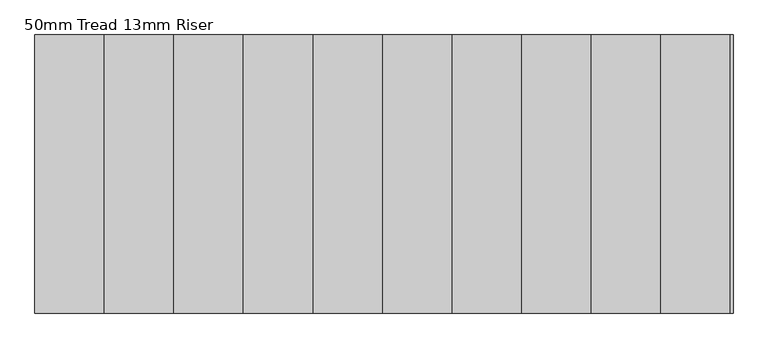
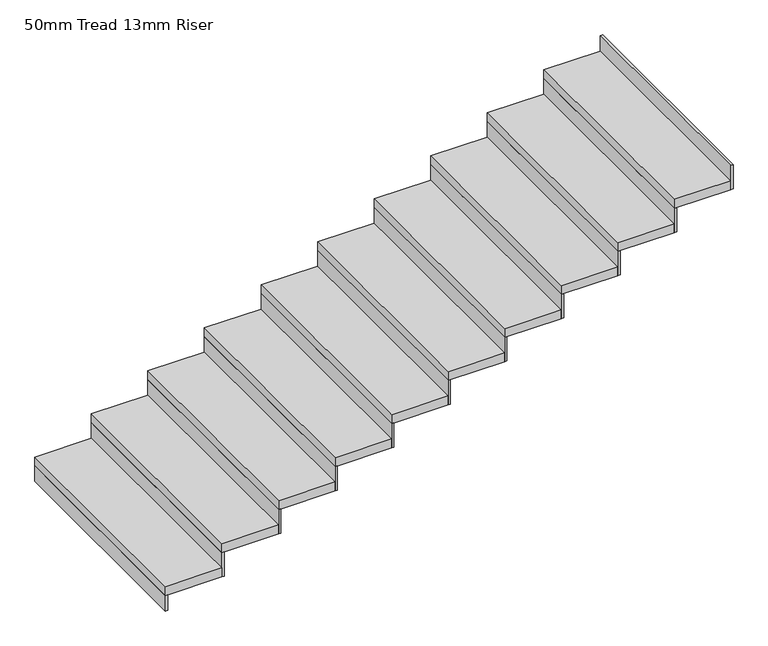
"""IFC4 building model written with IfcOpenShell, lengths in millimetres: stair flight geometry, 50mm Tread 13mm Riser."""

from ifc_helpers import new_model, si_unit, frame, origin, origin_with_axes, place, context, project, spatial, polyline, outline, extrude, source, transform, mapped, element, save


def stair_flight_50mm_tread_13mm_riser_f56aad4f(model_context):
    return source(origin(), model_context, "Body", "SweptSolid", [
        extrude(outline(polyline([(-12061.9417114, -7269.8807746), (-12074.4417114, -7269.8807746), (-12074.4417114, -6069.8807746), (-12061.9417114, -6069.8807746), (-12061.9417114, -7269.8807746)])), origin_with_axes(), (0.0, 0.0, 1.0), 86.3636364),
        extrude(outline(polyline([(-11774.4417114, -6069.8807746), (-11774.4417114, -7269.8807746), (-12074.4417114, -7269.8807746), (-12074.4417114, -6069.8807746), (-11774.4417114, -6069.8807746)])), frame((0.0, 0.0, 86.3636364), z_axis=(0.0, 0.0, 1.0), x_axis=(1.0, 0.0, 0.0)), (0.0, 0.0, 1.0), 50.0),
        extrude(outline(polyline([(-11761.9417114, -7269.8807746), (-11774.4417114, -7269.8807746), (-11774.4417114, -6069.8807746), (-11761.9417114, -6069.8807746), (-11761.9417114, -7269.8807746)])), frame((0.0, 0.0, 86.3636364), z_axis=(0.0, 0.0, 1.0), x_axis=(1.0, 0.0, 0.0)), (0.0, 0.0, 1.0), 136.3636364),
        extrude(outline(polyline([(-11474.4417114, -6069.8807746), (-11474.4417114, -7269.8807746), (-11774.4417114, -7269.8807746), (-11774.4417114, -6069.8807746), (-11474.4417114, -6069.8807746)])), frame((0.0, 0.0, 222.7272727), z_axis=(0.0, 0.0, 1.0), x_axis=(1.0, 0.0, 0.0)), (0.0, 0.0, 1.0), 50.0),
        extrude(outline(polyline([(-11461.9417114, -7269.8807746), (-11474.4417114, -7269.8807746), (-11474.4417114, -6069.8807746), (-11461.9417114, -6069.8807746), (-11461.9417114, -7269.8807746)])), frame((0.0, 0.0, 222.7272727), z_axis=(0.0, 0.0, 1.0), x_axis=(1.0, 0.0, 0.0)), (0.0, 0.0, 1.0), 136.3636364),
        extrude(outline(polyline([(-11174.4417114, -6069.8807746), (-11174.4417114, -7269.8807746), (-11474.4417114, -7269.8807746), (-11474.4417114, -6069.8807746), (-11174.4417114, -6069.8807746)])), frame((0.0, 0.0, 359.0909091), z_axis=(0.0, 0.0, 1.0), x_axis=(1.0, 0.0, 0.0)), (0.0, 0.0, 1.0), 50.0),
        extrude(outline(polyline([(-11161.9417114, -7269.8807746), (-11174.4417114, -7269.8807746), (-11174.4417114, -6069.8807746), (-11161.9417114, -6069.8807746), (-11161.9417114, -7269.8807746)])), frame((0.0, 0.0, 359.0909091), z_axis=(0.0, 0.0, 1.0), x_axis=(1.0, 0.0, 0.0)), (0.0, 0.0, 1.0), 136.3636364),
        extrude(outline(polyline([(-10874.4417114, -6069.8807746), (-10874.4417114, -7269.8807746), (-11174.4417114, -7269.8807746), (-11174.4417114, -6069.8807746), (-10874.4417114, -6069.8807746)])), frame((0.0, 0.0, 495.4545455), z_axis=(0.0, 0.0, 1.0), x_axis=(1.0, 0.0, 0.0)), (0.0, 0.0, 1.0), 50.0),
        extrude(outline(polyline([(-10861.9417114, -7269.8807746), (-10874.4417114, -7269.8807746), (-10874.4417114, -6069.8807746), (-10861.9417114, -6069.8807746), (-10861.9417114, -7269.8807746)])), frame((0.0, 0.0, 495.4545455), z_axis=(0.0, 0.0, 1.0), x_axis=(1.0, 0.0, 0.0)), (0.0, 0.0, 1.0), 136.3636364),
        extrude(outline(polyline([(-10574.4417114, -6069.8807746), (-10574.4417114, -7269.8807746), (-10874.4417114, -7269.8807746), (-10874.4417114, -6069.8807746), (-10574.4417114, -6069.8807746)])), frame((0.0, 0.0, 631.8181818), z_axis=(0.0, 0.0, 1.0), x_axis=(1.0, 0.0, 0.0)), (0.0, 0.0, 1.0), 50.0),
        extrude(outline(polyline([(-10561.9417114, -7269.8807746), (-10574.4417114, -7269.8807746), (-10574.4417114, -6069.8807746), (-10561.9417114, -6069.8807746), (-10561.9417114, -7269.8807746)])), frame((0.0, 0.0, 631.8181818), z_axis=(0.0, 0.0, 1.0), x_axis=(1.0, 0.0, 0.0)), (0.0, 0.0, 1.0), 136.3636364),
        extrude(outline(polyline([(-10274.4417114, -6069.8807746), (-10274.4417114, -7269.8807746), (-10574.4417114, -7269.8807746), (-10574.4417114, -6069.8807746), (-10274.4417114, -6069.8807746)])), frame((0.0, 0.0, 768.1818182), z_axis=(0.0, 0.0, 1.0), x_axis=(1.0, 0.0, 0.0)), (0.0, 0.0, 1.0), 50.0),
        extrude(outline(polyline([(-10261.9417114, -7269.8807746), (-10274.4417114, -7269.8807746), (-10274.4417114, -6069.8807746), (-10261.9417114, -6069.8807746), (-10261.9417114, -7269.8807746)])), frame((0.0, 0.0, 768.1818182), z_axis=(0.0, 0.0, 1.0), x_axis=(1.0, 0.0, 0.0)), (0.0, 0.0, 1.0), 136.3636364),
        extrude(outline(polyline([(-9974.4417114, -6069.8807746), (-9974.4417114, -7269.8807746), (-10274.4417114, -7269.8807746), (-10274.4417114, -6069.8807746), (-9974.4417114, -6069.8807746)])), frame((0.0, 0.0, 904.5454545), z_axis=(0.0, 0.0, 1.0), x_axis=(1.0, 0.0, 0.0)), (0.0, 0.0, 1.0), 50.0),
        extrude(outline(polyline([(-9961.9417114, -7269.8807746), (-9974.4417114, -7269.8807746), (-9974.4417114, -6069.8807746), (-9961.9417114, -6069.8807746), (-9961.9417114, -7269.8807746)])), frame((0.0, 0.0, 904.5454545), z_axis=(0.0, 0.0, 1.0), x_axis=(1.0, 0.0, 0.0)), (0.0, 0.0, 1.0), 136.3636364),
        extrude(outline(polyline([(-9674.4417114, -6069.8807746), (-9674.4417114, -7269.8807746), (-9974.4417114, -7269.8807746), (-9974.4417114, -6069.8807746), (-9674.4417114, -6069.8807746)])), frame((0.0, 0.0, 1040.9090909), z_axis=(0.0, 0.0, 1.0), x_axis=(1.0, 0.0, 0.0)), (0.0, 0.0, 1.0), 50.0),
        extrude(outline(polyline([(-9661.9417114, -7269.8807746), (-9674.4417114, -7269.8807746), (-9674.4417114, -6069.8807746), (-9661.9417114, -6069.8807746), (-9661.9417114, -7269.8807746)])), frame((0.0, 0.0, 1040.9090909), z_axis=(0.0, 0.0, 1.0), x_axis=(1.0, 0.0, 0.0)), (0.0, 0.0, 1.0), 136.3636364),
        extrude(outline(polyline([(-9374.4417114, -6069.8807746), (-9374.4417114, -7269.8807746), (-9674.4417114, -7269.8807746), (-9674.4417114, -6069.8807746), (-9374.4417114, -6069.8807746)])), frame((0.0, 0.0, 1177.2727273), z_axis=(0.0, 0.0, 1.0), x_axis=(1.0, 0.0, 0.0)), (0.0, 0.0, 1.0), 50.0),
        extrude(outline(polyline([(-9361.9417114, -7269.8807746), (-9374.4417114, -7269.8807746), (-9374.4417114, -6069.8807746), (-9361.9417114, -6069.8807746), (-9361.9417114, -7269.8807746)])), frame((0.0, 0.0, 1177.2727273), z_axis=(0.0, 0.0, 1.0), x_axis=(1.0, 0.0, 0.0)), (0.0, 0.0, 1.0), 136.3636364),
        extrude(outline(polyline([(-9061.9417114, -7269.8807746), (-9074.4417114, -7269.8807746), (-9074.4417114, -6069.8807746), (-9061.9417114, -6069.8807746), (-9061.9417114, -7269.8807746)])), frame((0.0, 0.0, 1313.6363636), z_axis=(0.0, 0.0, 1.0), x_axis=(1.0, 0.0, 0.0)), (0.0, 0.0, 1.0), 136.3636364),
        extrude(outline(polyline([(-9074.4417114, -6069.8807746), (-9074.4417114, -7269.8807746), (-9374.4417114, -7269.8807746), (-9374.4417114, -6069.8807746), (-9074.4417114, -6069.8807746)])), frame((0.0, 0.0, 1313.6363636), z_axis=(0.0, 0.0, 1.0), x_axis=(1.0, 0.0, 0.0)), (0.0, 0.0, 1.0), 50.0),
    ])


if __name__ == "__main__":
    model = new_model("IFC4")
    model_context = context("Model", 3, world=origin())
    ifc_project = project(units=[si_unit("LENGTHUNIT", "METRE", prefix="MILLI")], contexts=[model_context])
    site = spatial("IfcSite", under=ifc_project)
    building = spatial("IfcBuilding", under=site)
    placement = place(None, origin())
    stair_flight_50mm_tread_13mm_riser_shape = stair_flight_50mm_tread_13mm_riser_f56aad4f(model_context)
    element("IfcStairFlight", 1, ObjectType="50mm Tread 13mm Riser", at=placement, inside=building, context=model_context, shape_type="MappedRepresentation", body=[
        mapped(stair_flight_50mm_tread_13mm_riser_shape, transform((0.0, 0.0, 0.0), x_axis=(1.0, 0.0, 0.0), y_axis=(0.0, 1.0, 0.0), z_axis=(0.0, 0.0, 1.0))),
    ])
    save(model, "model.ifc")
